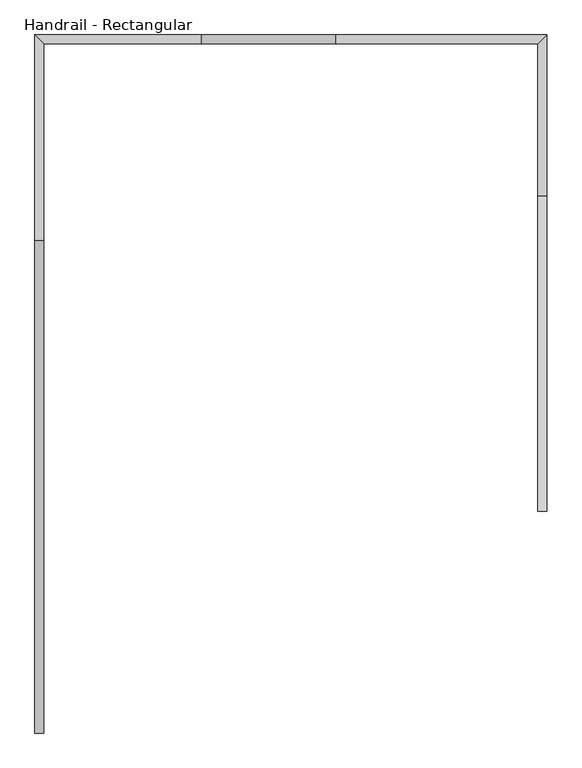
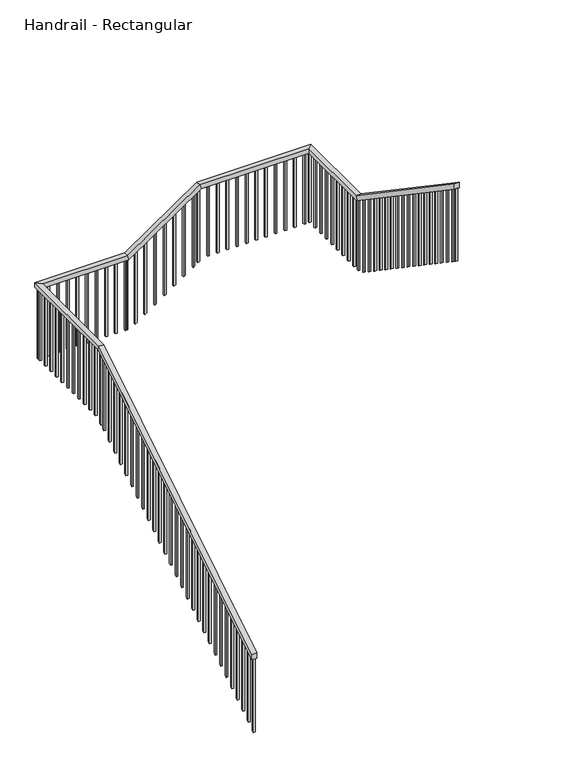
"""IFC4 building model written with IfcOpenShell, lengths in millimetres: railing geometry, Handrail - Rectangular."""

from ifc_helpers import new_model, si_unit, frame, origin, place, context, project, spatial, polyline, outline, extrude, faceted_brep, source, transform, mapped, element, save


def handrail_rectangular_2ff46d95(model_context):
    return source(origin(), model_context, "Body", "SolidModel", [
        faceted_brep([(-5540.3586735, -1605.5757069, -2569.0285714), (-5540.3586735, -1605.5757069, -2628.8906848), (-5489.5586735, -1605.5757069, -2628.8906848), (-5489.5586735, -1605.5757069, -2569.0285714), (-5540.3586735, 1188.4242931, -827.3142857), (-5540.3586735, 1202.9614332, -878.1142857), (-5489.5586735, 1202.9614332, -878.1142857), (-5489.5586735, 1188.4242931, -827.3142857), (-5540.3586735, 2356.8242931, -827.3142857), (-5540.3586735, 2356.8242931, -878.1142857), (-5489.5586735, 2306.0242931, -878.1142857), (-5489.5586735, 2306.0242931, -827.3142857), (-4594.2086735, 2356.8242931, -827.3142857), (-4578.4645039, 2356.8242931, -878.1142857), (-4578.4645039, 2306.0242931, -878.1142857), (-4594.2086735, 2306.0242931, -827.3142857), (-3832.2086735, 2356.8242931, -304.8), (-3816.4645039, 2356.8242931, -355.6), (-3816.4645039, 2306.0242931, -355.6), (-3832.2086735, 2306.0242931, -304.8), (-2632.0586735, 2356.8242931, -304.8), (-2632.0586735, 2356.8242931, -355.6), (-2682.8586735, 2306.0242931, -355.6), (-2682.8586735, 2306.0242931, -304.8), (-2632.0586735, 1444.5409597, -304.8), (-2632.0586735, 1428.9043211, -355.6), (-2682.8586735, 1428.9043211, -355.6), (-2682.8586735, 1444.5409597, -304.8), (-2632.0586735, -348.2757069, 914.4), (-2682.8586735, -348.2757069, 914.4), (-2682.8586735, -348.2757069, 852.9663473), (-2632.0586735, -348.2757069, 852.9663473)], [[[0, 1, 2, 3]], [[1, 0, 4, 5]], [[2, 1, 5, 6]], [[3, 2, 6, 7]], [[0, 3, 7, 4]], [[5, 4, 8, 9]], [[6, 5, 9, 10]], [[7, 6, 10, 11]], [[4, 7, 11, 8]], [[9, 8, 12, 13]], [[10, 9, 13, 14]], [[11, 10, 14, 15]], [[8, 11, 15, 12]], [[13, 12, 16, 17]], [[14, 13, 17, 18]], [[15, 14, 18, 19]], [[12, 15, 19, 16]], [[17, 16, 20, 21]], [[18, 17, 21, 22]], [[19, 18, 22, 23]], [[16, 19, 23, 20]], [[21, 20, 24, 25]], [[22, 21, 25, 26]], [[23, 22, 26, 27]], [[20, 23, 27, 24]], [[28, 29, 30, 31]], [[25, 24, 28, 31]], [[26, 25, 31, 30]], [[27, 26, 30, 29]], [[24, 27, 29, 28]]]),
        extrude(outline(polyline([(-273.1340403, 801.8664653), (-273.1340403, -5.8529595), (-292.1840403, 7.1019402), (-292.1840403, 814.821365), (-273.1340403, 801.8664653)])), frame((-2666.9836735, 0.0, 0.0), z_axis=(1.0, 0.0, 0.0), x_axis=(0.0, 1.0, 0.0)), (0.0, 0.0, 1.0), 19.05),
        extrude(outline(polyline([(-171.5340403, 732.7736672), (-171.5340403, -74.9457576), (-190.5840403, -61.9908579), (-190.5840403, 745.7285669), (-171.5340403, 732.7736672)])), frame((-2666.9836735, 0.0, 0.0), z_axis=(1.0, 0.0, 0.0), x_axis=(0.0, 1.0, 0.0)), (0.0, 0.0, 1.0), 19.05),
        extrude(outline(polyline([(-69.9340403, 663.6808691), (-69.9340403, -144.0385557), (-88.9840403, -131.083656), (-88.9840403, 676.6357688), (-69.9340403, 663.6808691)])), frame((-2666.9836735, 0.0, 0.0), z_axis=(1.0, 0.0, 0.0), x_axis=(0.0, 1.0, 0.0)), (0.0, 0.0, 1.0), 19.05),
        extrude(outline(polyline([(31.6659597, 594.588071), (31.6659597, -213.1313538), (12.6159597, -200.1764541), (12.6159597, 607.5429706), (31.6659597, 594.588071)])), frame((-2666.9836735, 0.0, 0.0), z_axis=(1.0, 0.0, 0.0), x_axis=(0.0, 1.0, 0.0)), (0.0, 0.0, 1.0), 19.05),
        extrude(outline(polyline([(133.2659597, 525.4952729), (133.2659597, -282.2241519), (114.2159597, -269.2692522), (114.2159597, 538.4501725), (133.2659597, 525.4952729)])), frame((-2666.9836735, 0.0, 0.0), z_axis=(1.0, 0.0, 0.0), x_axis=(0.0, 1.0, 0.0)), (0.0, 0.0, 1.0), 19.05),
        extrude(outline(polyline([(234.8659597, 456.4024748), (234.8659597, -351.31695), (215.8159597, -338.3620504), (215.8159597, 469.3573744), (234.8659597, 456.4024748)])), frame((-2666.9836735, 0.0, 0.0), z_axis=(1.0, 0.0, 0.0), x_axis=(0.0, 1.0, 0.0)), (0.0, 0.0, 1.0), 19.05),
        extrude(outline(polyline([(336.4659597, 387.3096767), (336.4659597, -420.4097481), (317.4159597, -407.4548485), (317.4159597, 400.2645763), (336.4659597, 387.3096767)])), frame((-2666.9836735, 0.0, 0.0), z_axis=(1.0, 0.0, 0.0), x_axis=(0.0, 1.0, 0.0)), (0.0, 0.0, 1.0), 19.05),
        extrude(outline(polyline([(438.0659597, 318.2168786), (438.0659597, -489.5025462), (419.0159597, -476.5476466), (419.0159597, 331.1717782), (438.0659597, 318.2168786)])), frame((-2666.9836735, 0.0, 0.0), z_axis=(1.0, 0.0, 0.0), x_axis=(0.0, 1.0, 0.0)), (0.0, 0.0, 1.0), 19.05),
        extrude(outline(polyline([(539.6659597, 249.1240804), (539.6659597, -558.5953443), (520.6159597, -545.6404447), (520.6159597, 262.0789801), (539.6659597, 249.1240804)])), frame((-2666.9836735, 0.0, 0.0), z_axis=(1.0, 0.0, 0.0), x_axis=(0.0, 1.0, 0.0)), (0.0, 0.0, 1.0), 19.05),
        extrude(outline(polyline([(641.2659597, 180.0312823), (641.2659597, -627.6881425), (622.2159597, -614.7332428), (622.2159597, 192.986182), (641.2659597, 180.0312823)])), frame((-2666.9836735, 0.0, 0.0), z_axis=(1.0, 0.0, 0.0), x_axis=(0.0, 1.0, 0.0)), (0.0, 0.0, 1.0), 19.05),
        extrude(outline(polyline([(742.8659597, 110.9384842), (742.8659597, -696.7809406), (723.8159597, -683.8260409), (723.8159597, 123.8933839), (742.8659597, 110.9384842)])), frame((-2666.9836735, 0.0, 0.0), z_axis=(1.0, 0.0, 0.0), x_axis=(0.0, 1.0, 0.0)), (0.0, 0.0, 1.0), 19.05),
        extrude(outline(polyline([(844.4659597, 41.8456861), (844.4659597, -765.8737387), (825.4159597, -752.918839), (825.4159597, 54.8005858), (844.4659597, 41.8456861)])), frame((-2666.9836735, 0.0, 0.0), z_axis=(1.0, 0.0, 0.0), x_axis=(0.0, 1.0, 0.0)), (0.0, 0.0, 1.0), 19.05),
        extrude(outline(polyline([(946.0659597, -27.247112), (946.0659597, -834.9665368), (927.0159597, -822.0116371), (927.0159597, -14.2922124), (946.0659597, -27.247112)])), frame((-2666.9836735, 0.0, 0.0), z_axis=(1.0, 0.0, 0.0), x_axis=(0.0, 1.0, 0.0)), (0.0, 0.0, 1.0), 19.05),
        extrude(outline(polyline([(1047.6659597, -96.3399101), (1047.6659597, -904.0593349), (1028.6159597, -891.1044352), (1028.6159597, -83.3850105), (1047.6659597, -96.3399101)])), frame((-2666.9836735, 0.0, 0.0), z_axis=(1.0, 0.0, 0.0), x_axis=(0.0, 1.0, 0.0)), (0.0, 0.0, 1.0), 19.05),
        extrude(outline(polyline([(1149.2659597, -165.4327082), (1149.2659597, -973.152133), (1130.2159597, -960.1972334), (1130.2159597, -152.4778086), (1149.2659597, -165.4327082)])), frame((-2666.9836735, 0.0, 0.0), z_axis=(1.0, 0.0, 0.0), x_axis=(0.0, 1.0, 0.0)), (0.0, 0.0, 1.0), 19.05),
        extrude(outline(polyline([(1250.8659597, -234.5255063), (1250.8659597, -1042.2449311), (1231.8159597, -1029.2900315), (1231.8159597, -221.5706067), (1250.8659597, -234.5255063)])), frame((-2666.9836735, 0.0, 0.0), z_axis=(1.0, 0.0, 0.0), x_axis=(0.0, 1.0, 0.0)), (0.0, 0.0, 1.0), 19.05),
        extrude(outline(polyline([(1352.4659597, -303.6183044), (1352.4659597, -1111.3377292), (1333.4159597, -1098.3828296), (1333.4159597, -290.6634048), (1352.4659597, -303.6183044)])), frame((-2666.9836735, 0.0, 0.0), z_axis=(1.0, 0.0, 0.0), x_axis=(0.0, 1.0, 0.0)), (0.0, 0.0, 1.0), 19.05),
        extrude(outline(polyline([(-2647.9336735, 1528.1492931), (-2647.9336735, 1509.0992931), (-2666.9836735, 1509.0992931), (-2666.9836735, 1528.1492931), (-2647.9336735, 1528.1492931)])), frame((0.0, 0.0, -1143.0), z_axis=(0.0, 0.0, 1.0), x_axis=(1.0, 0.0, 0.0)), (0.0, 0.0, 1.0), 787.4),
        extrude(outline(polyline([(-2647.9336735, 1629.7492931), (-2647.9336735, 1610.6992931), (-2666.9836735, 1610.6992931), (-2666.9836735, 1629.7492931), (-2647.9336735, 1629.7492931)])), frame((0.0, 0.0, -1143.0), z_axis=(0.0, 0.0, 1.0), x_axis=(1.0, 0.0, 0.0)), (0.0, 0.0, 1.0), 787.4),
        extrude(outline(polyline([(-2647.9336735, 1731.3492931), (-2647.9336735, 1712.2992931), (-2666.9836735, 1712.2992931), (-2666.9836735, 1731.3492931), (-2647.9336735, 1731.3492931)])), frame((0.0, 0.0, -1143.0), z_axis=(0.0, 0.0, 1.0), x_axis=(1.0, 0.0, 0.0)), (0.0, 0.0, 1.0), 787.4),
        extrude(outline(polyline([(-2647.9336735, 1832.9492931), (-2647.9336735, 1813.8992931), (-2666.9836735, 1813.8992931), (-2666.9836735, 1832.9492931), (-2647.9336735, 1832.9492931)])), frame((0.0, 0.0, -1143.0), z_axis=(0.0, 0.0, 1.0), x_axis=(1.0, 0.0, 0.0)), (0.0, 0.0, 1.0), 787.4),
        extrude(outline(polyline([(-2647.9336735, 1934.5492931), (-2647.9336735, 1915.4992931), (-2666.9836735, 1915.4992931), (-2666.9836735, 1934.5492931), (-2647.9336735, 1934.5492931)])), frame((0.0, 0.0, -1143.0), z_axis=(0.0, 0.0, 1.0), x_axis=(1.0, 0.0, 0.0)), (0.0, 0.0, 1.0), 787.4),
        extrude(outline(polyline([(-2647.9336735, 2036.1492931), (-2647.9336735, 2017.0992931), (-2666.9836735, 2017.0992931), (-2666.9836735, 2036.1492931), (-2647.9336735, 2036.1492931)])), frame((0.0, 0.0, -1143.0), z_axis=(0.0, 0.0, 1.0), x_axis=(1.0, 0.0, 0.0)), (0.0, 0.0, 1.0), 787.4),
        extrude(outline(polyline([(-2647.9336735, 2137.7492931), (-2647.9336735, 2118.6992931), (-2666.9836735, 2118.6992931), (-2666.9836735, 2137.7492931), (-2647.9336735, 2137.7492931)])), frame((0.0, 0.0, -1143.0), z_axis=(0.0, 0.0, 1.0), x_axis=(1.0, 0.0, 0.0)), (0.0, 0.0, 1.0), 787.4),
        extrude(outline(polyline([(-2647.9336735, 2239.3492931), (-2647.9336735, 2220.2992931), (-2666.9836735, 2220.2992931), (-2666.9836735, 2239.3492931), (-2647.9336735, 2239.3492931)])), frame((0.0, 0.0, -1143.0), z_axis=(0.0, 0.0, 1.0), x_axis=(1.0, 0.0, 0.0)), (0.0, 0.0, 1.0), 787.4),
        extrude(outline(polyline([(-2724.1336735, 2340.9492931), (-2705.0836735, 2340.9492931), (-2705.0836735, 2321.8992931), (-2724.1336735, 2321.8992931), (-2724.1336735, 2340.9492931)])), frame((0.0, 0.0, -1143.0), z_axis=(0.0, 0.0, 1.0), x_axis=(1.0, 0.0, 0.0)), (0.0, 0.0, 1.0), 787.4),
        extrude(outline(polyline([(-2825.7336735, 2340.9492931), (-2806.6836735, 2340.9492931), (-2806.6836735, 2321.8992931), (-2825.7336735, 2321.8992931), (-2825.7336735, 2340.9492931)])), frame((0.0, 0.0, -1143.0), z_axis=(0.0, 0.0, 1.0), x_axis=(1.0, 0.0, 0.0)), (0.0, 0.0, 1.0), 787.4),
        extrude(outline(polyline([(-2927.3336735, 2340.9492931), (-2908.2836735, 2340.9492931), (-2908.2836735, 2321.8992931), (-2927.3336735, 2321.8992931), (-2927.3336735, 2340.9492931)])), frame((0.0, 0.0, -1143.0), z_axis=(0.0, 0.0, 1.0), x_axis=(1.0, 0.0, 0.0)), (0.0, 0.0, 1.0), 787.4),
        extrude(outline(polyline([(-3028.9336735, 2340.9492931), (-3009.8836735, 2340.9492931), (-3009.8836735, 2321.8992931), (-3028.9336735, 2321.8992931), (-3028.9336735, 2340.9492931)])), frame((0.0, 0.0, -1143.0), z_axis=(0.0, 0.0, 1.0), x_axis=(1.0, 0.0, 0.0)), (0.0, 0.0, 1.0), 787.4),
        extrude(outline(polyline([(-3130.5336735, 2340.9492931), (-3111.4836735, 2340.9492931), (-3111.4836735, 2321.8992931), (-3130.5336735, 2321.8992931), (-3130.5336735, 2340.9492931)])), frame((0.0, 0.0, -1143.0), z_axis=(0.0, 0.0, 1.0), x_axis=(1.0, 0.0, 0.0)), (0.0, 0.0, 1.0), 787.4),
        extrude(outline(polyline([(-3232.1336735, 2340.9492931), (-3213.0836735, 2340.9492931), (-3213.0836735, 2321.8992931), (-3232.1336735, 2321.8992931), (-3232.1336735, 2340.9492931)])), frame((0.0, 0.0, -1143.0), z_axis=(0.0, 0.0, 1.0), x_axis=(1.0, 0.0, 0.0)), (0.0, 0.0, 1.0), 787.4),
        extrude(outline(polyline([(-3333.7336735, 2340.9492931), (-3314.6836735, 2340.9492931), (-3314.6836735, 2321.8992931), (-3333.7336735, 2321.8992931), (-3333.7336735, 2340.9492931)])), frame((0.0, 0.0, -1143.0), z_axis=(0.0, 0.0, 1.0), x_axis=(1.0, 0.0, 0.0)), (0.0, 0.0, 1.0), 787.4),
        extrude(outline(polyline([(-3435.3336735, 2340.9492931), (-3416.2836735, 2340.9492931), (-3416.2836735, 2321.8992931), (-3435.3336735, 2321.8992931), (-3435.3336735, 2340.9492931)])), frame((0.0, 0.0, -1143.0), z_axis=(0.0, 0.0, 1.0), x_axis=(1.0, 0.0, 0.0)), (0.0, 0.0, 1.0), 787.4),
        extrude(outline(polyline([(-3536.9336735, 2340.9492931), (-3517.8836735, 2340.9492931), (-3517.8836735, 2321.8992931), (-3536.9336735, 2321.8992931), (-3536.9336735, 2340.9492931)])), frame((0.0, 0.0, -1143.0), z_axis=(0.0, 0.0, 1.0), x_axis=(1.0, 0.0, 0.0)), (0.0, 0.0, 1.0), 787.4),
        extrude(outline(polyline([(-3638.5336735, 2340.9492931), (-3619.4836735, 2340.9492931), (-3619.4836735, 2321.8992931), (-3638.5336735, 2321.8992931), (-3638.5336735, 2340.9492931)])), frame((0.0, 0.0, -1143.0), z_axis=(0.0, 0.0, 1.0), x_axis=(1.0, 0.0, 0.0)), (0.0, 0.0, 1.0), 787.4),
        extrude(outline(polyline([(-3740.1336735, 2340.9492931), (-3721.0836735, 2340.9492931), (-3721.0836735, 2321.8992931), (-3740.1336735, 2321.8992931), (-3740.1336735, 2340.9492931)])), frame((0.0, 0.0, -1143.0), z_axis=(0.0, 0.0, 1.0), x_axis=(1.0, 0.0, 0.0)), (0.0, 0.0, 1.0), 787.4),
        extrude(outline(polyline([(-407.7617163, -3892.5336735), (-1214.727562, -3892.5336735), (-1201.6647048, -3873.4836735), (-394.6988591, -3873.4836735), (-407.7617163, -3892.5336735)])), frame((0.0, 2321.8992931, 0.0), z_axis=(0.0, 1.0, 0.0), x_axis=(0.0, 0.0, 1.0)), (0.0, 0.0, 1.0), 19.05),
        extrude(outline(polyline([(-477.4302877, -3994.1336735), (-1284.3961334, -3994.1336735), (-1271.3332763, -3975.0836735), (-464.3674306, -3975.0836735), (-477.4302877, -3994.1336735)])), frame((0.0, 2321.8992931, 0.0), z_axis=(0.0, 1.0, 0.0), x_axis=(0.0, 0.0, 1.0)), (0.0, 0.0, 1.0), 19.05),
        extrude(outline(polyline([(-547.0988591, -4095.7336735), (-1354.0647048, -4095.7336735), (-1341.0018477, -4076.6836735), (-534.036002, -4076.6836735), (-547.0988591, -4095.7336735)])), frame((0.0, 2321.8992931, 0.0), z_axis=(0.0, 1.0, 0.0), x_axis=(0.0, 0.0, 1.0)), (0.0, 0.0, 1.0), 19.05),
        extrude(outline(polyline([(-616.7674306, -4197.3336735), (-1423.7332763, -4197.3336735), (-1410.6704191, -4178.2836735), (-603.7045734, -4178.2836735), (-616.7674306, -4197.3336735)])), frame((0.0, 2321.8992931, 0.0), z_axis=(0.0, 1.0, 0.0), x_axis=(0.0, 0.0, 1.0)), (0.0, 0.0, 1.0), 19.05),
        extrude(outline(polyline([(-686.436002, -4298.9336735), (-1493.4018477, -4298.9336735), (-1480.3389905, -4279.8836735), (-673.3731448, -4279.8836735), (-686.436002, -4298.9336735)])), frame((0.0, 2321.8992931, 0.0), z_axis=(0.0, 1.0, 0.0), x_axis=(0.0, 0.0, 1.0)), (0.0, 0.0, 1.0), 19.05),
        extrude(outline(polyline([(-756.1045734, -4400.5336735), (-1563.0704191, -4400.5336735), (-1550.007562, -4381.4836735), (-743.0417163, -4381.4836735), (-756.1045734, -4400.5336735)])), frame((0.0, 2321.8992931, 0.0), z_axis=(0.0, 1.0, 0.0), x_axis=(0.0, 0.0, 1.0)), (0.0, 0.0, 1.0), 19.05),
        extrude(outline(polyline([(-825.7731448, -4502.1336735), (-1632.7389905, -4502.1336735), (-1619.6761334, -4483.0836735), (-812.7102877, -4483.0836735), (-825.7731448, -4502.1336735)])), frame((0.0, 2321.8992931, 0.0), z_axis=(0.0, 1.0, 0.0), x_axis=(0.0, 0.0, 1.0)), (0.0, 0.0, 1.0), 19.05),
        extrude(outline(polyline([(-4610.0836735, 2340.9492931), (-4591.0336735, 2340.9492931), (-4591.0336735, 2321.8992931), (-4610.0836735, 2321.8992931), (-4610.0836735, 2340.9492931)])), frame((0.0, 0.0, -1665.5142857), z_axis=(0.0, 0.0, 1.0), x_axis=(1.0, 0.0, 0.0)), (0.0, 0.0, 1.0), 787.4),
        extrude(outline(polyline([(-4711.6836735, 2340.9492931), (-4692.6336735, 2340.9492931), (-4692.6336735, 2321.8992931), (-4711.6836735, 2321.8992931), (-4711.6836735, 2340.9492931)])), frame((0.0, 0.0, -1665.5142857), z_axis=(0.0, 0.0, 1.0), x_axis=(1.0, 0.0, 0.0)), (0.0, 0.0, 1.0), 787.4),
        extrude(outline(polyline([(-4813.2836735, 2340.9492931), (-4794.2336735, 2340.9492931), (-4794.2336735, 2321.8992931), (-4813.2836735, 2321.8992931), (-4813.2836735, 2340.9492931)])), frame((0.0, 0.0, -1665.5142857), z_axis=(0.0, 0.0, 1.0), x_axis=(1.0, 0.0, 0.0)), (0.0, 0.0, 1.0), 787.4),
        extrude(outline(polyline([(-4914.8836735, 2340.9492931), (-4895.8336735, 2340.9492931), (-4895.8336735, 2321.8992931), (-4914.8836735, 2321.8992931), (-4914.8836735, 2340.9492931)])), frame((0.0, 0.0, -1665.5142857), z_axis=(0.0, 0.0, 1.0), x_axis=(1.0, 0.0, 0.0)), (0.0, 0.0, 1.0), 787.4),
        extrude(outline(polyline([(-5016.4836735, 2340.9492931), (-4997.4336735, 2340.9492931), (-4997.4336735, 2321.8992931), (-5016.4836735, 2321.8992931), (-5016.4836735, 2340.9492931)])), frame((0.0, 0.0, -1665.5142857), z_axis=(0.0, 0.0, 1.0), x_axis=(1.0, 0.0, 0.0)), (0.0, 0.0, 1.0), 787.4),
        extrude(outline(polyline([(-5118.0836735, 2340.9492931), (-5099.0336735, 2340.9492931), (-5099.0336735, 2321.8992931), (-5118.0836735, 2321.8992931), (-5118.0836735, 2340.9492931)])), frame((0.0, 0.0, -1665.5142857), z_axis=(0.0, 0.0, 1.0), x_axis=(1.0, 0.0, 0.0)), (0.0, 0.0, 1.0), 787.4),
        extrude(outline(polyline([(-5219.6836735, 2340.9492931), (-5200.6336735, 2340.9492931), (-5200.6336735, 2321.8992931), (-5219.6836735, 2321.8992931), (-5219.6836735, 2340.9492931)])), frame((0.0, 0.0, -1665.5142857), z_axis=(0.0, 0.0, 1.0), x_axis=(1.0, 0.0, 0.0)), (0.0, 0.0, 1.0), 787.4),
        extrude(outline(polyline([(-5321.2836735, 2340.9492931), (-5302.2336735, 2340.9492931), (-5302.2336735, 2321.8992931), (-5321.2836735, 2321.8992931), (-5321.2836735, 2340.9492931)])), frame((0.0, 0.0, -1665.5142857), z_axis=(0.0, 0.0, 1.0), x_axis=(1.0, 0.0, 0.0)), (0.0, 0.0, 1.0), 787.4),
        extrude(outline(polyline([(-5422.8836735, 2340.9492931), (-5403.8336735, 2340.9492931), (-5403.8336735, 2321.8992931), (-5422.8836735, 2321.8992931), (-5422.8836735, 2340.9492931)])), frame((0.0, 0.0, -1665.5142857), z_axis=(0.0, 0.0, 1.0), x_axis=(1.0, 0.0, 0.0)), (0.0, 0.0, 1.0), 787.4),
        extrude(outline(polyline([(-5524.4836735, 2296.4992931), (-5524.4836735, 2315.5492931), (-5505.4336735, 2315.5492931), (-5505.4336735, 2296.4992931), (-5524.4836735, 2296.4992931)])), frame((0.0, 0.0, -1665.5142857), z_axis=(0.0, 0.0, 1.0), x_axis=(1.0, 0.0, 0.0)), (0.0, 0.0, 1.0), 787.4),
        extrude(outline(polyline([(-5524.4836735, 2194.8992931), (-5524.4836735, 2213.9492931), (-5505.4336735, 2213.9492931), (-5505.4336735, 2194.8992931), (-5524.4836735, 2194.8992931)])), frame((0.0, 0.0, -1665.5142857), z_axis=(0.0, 0.0, 1.0), x_axis=(1.0, 0.0, 0.0)), (0.0, 0.0, 1.0), 787.4),
        extrude(outline(polyline([(-5524.4836735, 2093.2992931), (-5524.4836735, 2112.3492931), (-5505.4336735, 2112.3492931), (-5505.4336735, 2093.2992931), (-5524.4836735, 2093.2992931)])), frame((0.0, 0.0, -1665.5142857), z_axis=(0.0, 0.0, 1.0), x_axis=(1.0, 0.0, 0.0)), (0.0, 0.0, 1.0), 787.4),
        extrude(outline(polyline([(-5524.4836735, 1991.6992931), (-5524.4836735, 2010.7492931), (-5505.4336735, 2010.7492931), (-5505.4336735, 1991.6992931), (-5524.4836735, 1991.6992931)])), frame((0.0, 0.0, -1665.5142857), z_axis=(0.0, 0.0, 1.0), x_axis=(1.0, 0.0, 0.0)), (0.0, 0.0, 1.0), 787.4),
        extrude(outline(polyline([(-5524.4836735, 1890.0992931), (-5524.4836735, 1909.1492931), (-5505.4336735, 1909.1492931), (-5505.4336735, 1890.0992931), (-5524.4836735, 1890.0992931)])), frame((0.0, 0.0, -1665.5142857), z_axis=(0.0, 0.0, 1.0), x_axis=(1.0, 0.0, 0.0)), (0.0, 0.0, 1.0), 787.4),
        extrude(outline(polyline([(-5524.4836735, 1788.4992931), (-5524.4836735, 1807.5492931), (-5505.4336735, 1807.5492931), (-5505.4336735, 1788.4992931), (-5524.4836735, 1788.4992931)])), frame((0.0, 0.0, -1665.5142857), z_axis=(0.0, 0.0, 1.0), x_axis=(1.0, 0.0, 0.0)), (0.0, 0.0, 1.0), 787.4),
        extrude(outline(polyline([(-5524.4836735, 1686.8992931), (-5524.4836735, 1705.9492931), (-5505.4336735, 1705.9492931), (-5505.4336735, 1686.8992931), (-5524.4836735, 1686.8992931)])), frame((0.0, 0.0, -1665.5142857), z_axis=(0.0, 0.0, 1.0), x_axis=(1.0, 0.0, 0.0)), (0.0, 0.0, 1.0), 787.4),
        extrude(outline(polyline([(-5524.4836735, 1585.2992931), (-5524.4836735, 1604.3492931), (-5505.4336735, 1604.3492931), (-5505.4336735, 1585.2992931), (-5524.4836735, 1585.2992931)])), frame((0.0, 0.0, -1665.5142857), z_axis=(0.0, 0.0, 1.0), x_axis=(1.0, 0.0, 0.0)), (0.0, 0.0, 1.0), 787.4),
        extrude(outline(polyline([(-5524.4836735, 1483.6992931), (-5524.4836735, 1502.7492931), (-5505.4336735, 1502.7492931), (-5505.4336735, 1483.6992931), (-5524.4836735, 1483.6992931)])), frame((0.0, 0.0, -1665.5142857), z_axis=(0.0, 0.0, 1.0), x_axis=(1.0, 0.0, 0.0)), (0.0, 0.0, 1.0), 787.4),
        extrude(outline(polyline([(-5524.4836735, 1382.0992931), (-5524.4836735, 1401.1492931), (-5505.4336735, 1401.1492931), (-5505.4336735, 1382.0992931), (-5524.4836735, 1382.0992931)])), frame((0.0, 0.0, -1665.5142857), z_axis=(0.0, 0.0, 1.0), x_axis=(1.0, 0.0, 0.0)), (0.0, 0.0, 1.0), 787.4),
        extrude(outline(polyline([(-5524.4836735, 1280.4992931), (-5524.4836735, 1299.5492931), (-5505.4336735, 1299.5492931), (-5505.4336735, 1280.4992931), (-5524.4836735, 1280.4992931)])), frame((0.0, 0.0, -1665.5142857), z_axis=(0.0, 0.0, 1.0), x_axis=(1.0, 0.0, 0.0)), (0.0, 0.0, 1.0), 787.4),
        extrude(outline(polyline([(1147.1492931, -912.9062692), (1147.1492931, -1727.8627539), (1128.0992931, -1739.7380786), (1128.0992931, -924.7815939), (1147.1492931, -912.9062692)])), frame((-5524.4836735, 0.0, 0.0), z_axis=(1.0, 0.0, 0.0), x_axis=(0.0, 1.0, 0.0)), (0.0, 0.0, 1.0), 19.05),
        extrude(outline(polyline([(1045.5492931, -976.2413341), (1045.5492931, -1791.1978188), (1026.4992931, -1803.0731435), (1026.4992931, -988.1166588), (1045.5492931, -976.2413341)])), frame((-5524.4836735, 0.0, 0.0), z_axis=(1.0, 0.0, 0.0), x_axis=(0.0, 1.0, 0.0)), (0.0, 0.0, 1.0), 19.05),
        extrude(outline(polyline([(943.9492931, -1039.576399), (943.9492931, -1854.5328838), (924.8992931, -1866.4082084), (924.8992931, -1051.4517237), (943.9492931, -1039.576399)])), frame((-5524.4836735, 0.0, 0.0), z_axis=(1.0, 0.0, 0.0), x_axis=(0.0, 1.0, 0.0)), (0.0, 0.0, 1.0), 19.05),
        extrude(outline(polyline([(842.3492931, -1102.911464), (842.3492931, -1917.8679487), (823.2992931, -1929.7432734), (823.2992931, -1114.7867887), (842.3492931, -1102.911464)])), frame((-5524.4836735, 0.0, 0.0), z_axis=(1.0, 0.0, 0.0), x_axis=(0.0, 1.0, 0.0)), (0.0, 0.0, 1.0), 19.05),
        extrude(outline(polyline([(740.7492931, -1166.2465289), (740.7492931, -1981.2030136), (721.6992931, -1993.0783383), (721.6992931, -1178.1218536), (740.7492931, -1166.2465289)])), frame((-5524.4836735, 0.0, 0.0), z_axis=(1.0, 0.0, 0.0), x_axis=(0.0, 1.0, 0.0)), (0.0, 0.0, 1.0), 19.05),
        extrude(outline(polyline([(639.1492931, -1229.5815939), (639.1492931, -2044.5380786), (620.0992931, -2056.4134032), (620.0992931, -1241.4569185), (639.1492931, -1229.5815939)])), frame((-5524.4836735, 0.0, 0.0), z_axis=(1.0, 0.0, 0.0), x_axis=(0.0, 1.0, 0.0)), (0.0, 0.0, 1.0), 19.05),
        extrude(outline(polyline([(537.5492931, -1292.9166588), (537.5492931, -2107.8731435), (518.4992931, -2119.7484682), (518.4992931, -1304.7919835), (537.5492931, -1292.9166588)])), frame((-5524.4836735, 0.0, 0.0), z_axis=(1.0, 0.0, 0.0), x_axis=(0.0, 1.0, 0.0)), (0.0, 0.0, 1.0), 19.05),
        extrude(outline(polyline([(435.9492931, -1356.2517237), (435.9492931, -2171.2082084), (416.8992931, -2183.0835331), (416.8992931, -1368.1270484), (435.9492931, -1356.2517237)])), frame((-5524.4836735, 0.0, 0.0), z_axis=(1.0, 0.0, 0.0), x_axis=(0.0, 1.0, 0.0)), (0.0, 0.0, 1.0), 19.05),
        extrude(outline(polyline([(334.3492931, -1419.5867887), (334.3492931, -2234.5432734), (315.2992931, -2246.418598), (315.2992931, -1431.4621133), (334.3492931, -1419.5867887)])), frame((-5524.4836735, 0.0, 0.0), z_axis=(1.0, 0.0, 0.0), x_axis=(0.0, 1.0, 0.0)), (0.0, 0.0, 1.0), 19.05),
        extrude(outline(polyline([(232.7492931, -1482.9218536), (232.7492931, -2297.8783383), (213.6992931, -2309.753663), (213.6992931, -1494.7971783), (232.7492931, -1482.9218536)])), frame((-5524.4836735, 0.0, 0.0), z_axis=(1.0, 0.0, 0.0), x_axis=(0.0, 1.0, 0.0)), (0.0, 0.0, 1.0), 19.05),
        extrude(outline(polyline([(131.1492931, -1546.2569185), (131.1492931, -2361.2134032), (112.0992931, -2373.0887279), (112.0992931, -1558.1322432), (131.1492931, -1546.2569185)])), frame((-5524.4836735, 0.0, 0.0), z_axis=(1.0, 0.0, 0.0), x_axis=(0.0, 1.0, 0.0)), (0.0, 0.0, 1.0), 19.05),
        extrude(outline(polyline([(29.5492931, -1609.5919835), (29.5492931, -2424.5484682), (10.4992931, -2436.4237928), (10.4992931, -1621.4673081), (29.5492931, -1609.5919835)])), frame((-5524.4836735, 0.0, 0.0), z_axis=(1.0, 0.0, 0.0), x_axis=(0.0, 1.0, 0.0)), (0.0, 0.0, 1.0), 19.05),
        extrude(outline(polyline([(-72.0507069, -1672.9270484), (-72.0507069, -2487.8835331), (-91.1007069, -2499.7588578), (-91.1007069, -1684.8023731), (-72.0507069, -1672.9270484)])), frame((-5524.4836735, 0.0, 0.0), z_axis=(1.0, 0.0, 0.0), x_axis=(0.0, 1.0, 0.0)), (0.0, 0.0, 1.0), 19.05),
        extrude(outline(polyline([(-173.6507069, -1736.2621133), (-173.6507069, -2551.218598), (-192.7007069, -2563.0939227), (-192.7007069, -1748.137438), (-173.6507069, -1736.2621133)])), frame((-5524.4836735, 0.0, 0.0), z_axis=(1.0, 0.0, 0.0), x_axis=(0.0, 1.0, 0.0)), (0.0, 0.0, 1.0), 19.05),
        extrude(outline(polyline([(-275.2507069, -1799.5971783), (-275.2507069, -2614.553663), (-294.3007069, -2626.4289876), (-294.3007069, -1811.4725029), (-275.2507069, -1799.5971783)])), frame((-5524.4836735, 0.0, 0.0), z_axis=(1.0, 0.0, 0.0), x_axis=(0.0, 1.0, 0.0)), (0.0, 0.0, 1.0), 19.05),
        extrude(outline(polyline([(-376.8507069, -1862.9322432), (-376.8507069, -2677.8887279), (-395.9007069, -2689.7640526), (-395.9007069, -1874.8075679), (-376.8507069, -1862.9322432)])), frame((-5524.4836735, 0.0, 0.0), z_axis=(1.0, 0.0, 0.0), x_axis=(0.0, 1.0, 0.0)), (0.0, 0.0, 1.0), 19.05),
        extrude(outline(polyline([(-478.4507069, -1926.2673081), (-478.4507069, -2741.2237928), (-497.5007069, -2753.0991175), (-497.5007069, -1938.1426328), (-478.4507069, -1926.2673081)])), frame((-5524.4836735, 0.0, 0.0), z_axis=(1.0, 0.0, 0.0), x_axis=(0.0, 1.0, 0.0)), (0.0, 0.0, 1.0), 19.05),
        extrude(outline(polyline([(-580.0507069, -1989.6023731), (-580.0507069, -2804.5588578), (-599.1007069, -2816.4341825), (-599.1007069, -2001.4776977), (-580.0507069, -1989.6023731)])), frame((-5524.4836735, 0.0, 0.0), z_axis=(1.0, 0.0, 0.0), x_axis=(0.0, 1.0, 0.0)), (0.0, 0.0, 1.0), 19.05),
        extrude(outline(polyline([(-681.6507069, -2052.937438), (-681.6507069, -2867.8939227), (-700.7007069, -2879.7692474), (-700.7007069, -2064.8127627), (-681.6507069, -2052.937438)])), frame((-5524.4836735, 0.0, 0.0), z_axis=(1.0, 0.0, 0.0), x_axis=(0.0, 1.0, 0.0)), (0.0, 0.0, 1.0), 19.05),
        extrude(outline(polyline([(-783.2507069, -2116.2725029), (-783.2507069, -2931.2289876), (-802.3007069, -2943.1043123), (-802.3007069, -2128.1478276), (-783.2507069, -2116.2725029)])), frame((-5524.4836735, 0.0, 0.0), z_axis=(1.0, 0.0, 0.0), x_axis=(0.0, 1.0, 0.0)), (0.0, 0.0, 1.0), 19.05),
        extrude(outline(polyline([(-884.8507069, -2179.6075679), (-884.8507069, -2994.5640526), (-903.9007069, -3006.4393773), (-903.9007069, -2191.4828926), (-884.8507069, -2179.6075679)])), frame((-5524.4836735, 0.0, 0.0), z_axis=(1.0, 0.0, 0.0), x_axis=(0.0, 1.0, 0.0)), (0.0, 0.0, 1.0), 19.05),
        extrude(outline(polyline([(-986.4507069, -2242.9426328), (-986.4507069, -3057.8991175), (-1005.5007069, -3069.7744422), (-1005.5007069, -2254.8179575), (-986.4507069, -2242.9426328)])), frame((-5524.4836735, 0.0, 0.0), z_axis=(1.0, 0.0, 0.0), x_axis=(0.0, 1.0, 0.0)), (0.0, 0.0, 1.0), 19.05),
        extrude(outline(polyline([(-1088.0507069, -2306.2776977), (-1088.0507069, -3121.2341825), (-1107.1007069, -3133.1095071), (-1107.1007069, -2318.1530224), (-1088.0507069, -2306.2776977)])), frame((-5524.4836735, 0.0, 0.0), z_axis=(1.0, 0.0, 0.0), x_axis=(0.0, 1.0, 0.0)), (0.0, 0.0, 1.0), 19.05),
        extrude(outline(polyline([(-1189.6507069, -2369.6127627), (-1189.6507069, -3184.5692474), (-1208.7007069, -3196.4445721), (-1208.7007069, -2381.4880874), (-1189.6507069, -2369.6127627)])), frame((-5524.4836735, 0.0, 0.0), z_axis=(1.0, 0.0, 0.0), x_axis=(0.0, 1.0, 0.0)), (0.0, 0.0, 1.0), 19.05),
        extrude(outline(polyline([(-1291.2507069, -2432.9478276), (-1291.2507069, -3247.9043123), (-1310.3007069, -3259.779637), (-1310.3007069, -2444.8231523), (-1291.2507069, -2432.9478276)])), frame((-5524.4836735, 0.0, 0.0), z_axis=(1.0, 0.0, 0.0), x_axis=(0.0, 1.0, 0.0)), (0.0, 0.0, 1.0), 19.05),
        extrude(outline(polyline([(-1392.8507069, -2496.2828926), (-1392.8507069, -3311.2393773), (-1411.9007069, -3323.1147019), (-1411.9007069, -2508.1582172), (-1392.8507069, -2496.2828926)])), frame((-5524.4836735, 0.0, 0.0), z_axis=(1.0, 0.0, 0.0), x_axis=(0.0, 1.0, 0.0)), (0.0, 0.0, 1.0), 19.05),
        extrude(outline(polyline([(-1494.4507069, -2559.6179575), (-1494.4507069, -3374.5744422), (-1513.5007069, -3386.4497669), (-1513.5007069, -2571.4932822), (-1494.4507069, -2559.6179575)])), frame((-5524.4836735, 0.0, 0.0), z_axis=(1.0, 0.0, 0.0), x_axis=(0.0, 1.0, 0.0)), (0.0, 0.0, 1.0), 19.05),
        extrude(outline(polyline([(-2647.9336735, 1454.0659597), (-2647.9336735, 1435.0159597), (-2666.9836735, 1435.0159597), (-2666.9836735, 1454.0659597), (-2647.9336735, 1454.0659597)])), frame((0.0, 0.0, -1143.0), z_axis=(0.0, 0.0, 1.0), x_axis=(1.0, 0.0, 0.0)), (0.0, 0.0, 1.0), 787.4),
        extrude(outline(polyline([(-2666.9836735, 2340.9492931), (-2647.9336735, 2340.9492931), (-2647.9336735, 2321.8992931), (-2666.9836735, 2321.8992931), (-2666.9836735, 2340.9492931)])), frame((0.0, 0.0, -1143.0), z_axis=(0.0, 0.0, 1.0), x_axis=(1.0, 0.0, 0.0)), (0.0, 0.0, 1.0), 787.4),
        extrude(outline(polyline([(-372.9274306, -3841.7336735), (-1179.8932763, -3841.7336735), (-1166.8304191, -3822.6836735), (-359.8645734, -3822.6836735), (-372.9274306, -3841.7336735)])), frame((0.0, 2321.8992931, 0.0), z_axis=(0.0, 1.0, 0.0), x_axis=(0.0, 0.0, 1.0)), (0.0, 0.0, 1.0), 19.05),
        extrude(outline(polyline([(-4603.7336735, 2340.9492931), (-4584.6836735, 2340.9492931), (-4584.6836735, 2321.8992931), (-4603.7336735, 2321.8992931), (-4603.7336735, 2340.9492931)])), frame((0.0, 0.0, -1665.5142857), z_axis=(0.0, 0.0, 1.0), x_axis=(1.0, 0.0, 0.0)), (0.0, 0.0, 1.0), 787.4),
        extrude(outline(polyline([(-5524.4836735, 2321.8992931), (-5524.4836735, 2340.9492931), (-5505.4336735, 2340.9492931), (-5505.4336735, 2321.8992931), (-5524.4836735, 2321.8992931)])), frame((0.0, 0.0, -1665.5142857), z_axis=(0.0, 0.0, 1.0), x_axis=(1.0, 0.0, 0.0)), (0.0, 0.0, 1.0), 787.4),
        extrude(outline(polyline([(1197.9492931, -881.2387367), (1197.9492931, -1696.1952214), (1178.8992931, -1708.0705461), (1178.8992931, -893.1140614), (1197.9492931, -881.2387367)])), frame((-5524.4836735, 0.0, 0.0), z_axis=(1.0, 0.0, 0.0), x_axis=(0.0, 1.0, 0.0)), (0.0, 0.0, 1.0), 19.05),
        extrude(outline(polyline([(-329.2257069, 840.0114476), (-329.2257069, 32.2920228), (-348.2757069, 45.2469225), (-348.2757069, 852.9663473), (-329.2257069, 840.0114476)])), frame((-2666.9836735, 0.0, 0.0), z_axis=(1.0, 0.0, 0.0), x_axis=(0.0, 1.0, 0.0)), (0.0, 0.0, 1.0), 19.05),
        extrude(outline(polyline([(-1586.5257069, -2617.0153601), (-1586.5257069, -3431.9718448), (-1605.5757069, -3443.8471695), (-1605.5757069, -2628.8906848), (-1586.5257069, -2617.0153601)])), frame((-5524.4836735, 0.0, 0.0), z_axis=(1.0, 0.0, 0.0), x_axis=(0.0, 1.0, 0.0)), (0.0, 0.0, 1.0), 19.05),
    ])


if __name__ == "__main__":
    model = new_model("IFC4")
    model_context = context("Model", 3, world=origin())
    ifc_project = project(units=[si_unit("LENGTHUNIT", "METRE", prefix="MILLI")], contexts=[model_context])
    site = spatial("IfcSite", under=ifc_project)
    building = spatial("IfcBuilding", under=site)
    placement = place(None, origin())
    handrail_rectangular_shape = handrail_rectangular_2ff46d95(model_context)
    element("IfcRailing", 1, ObjectType="Handrail - Rectangular", at=placement, inside=building, context=model_context, shape_type="MappedRepresentation", body=[
        mapped(handrail_rectangular_shape, transform((0.0, 0.0, 0.0), x_axis=(1.0, 0.0, 0.0), y_axis=(0.0, 1.0, 0.0), z_axis=(0.0, 0.0, 1.0))),
    ])
    save(model, "model.ifc")
